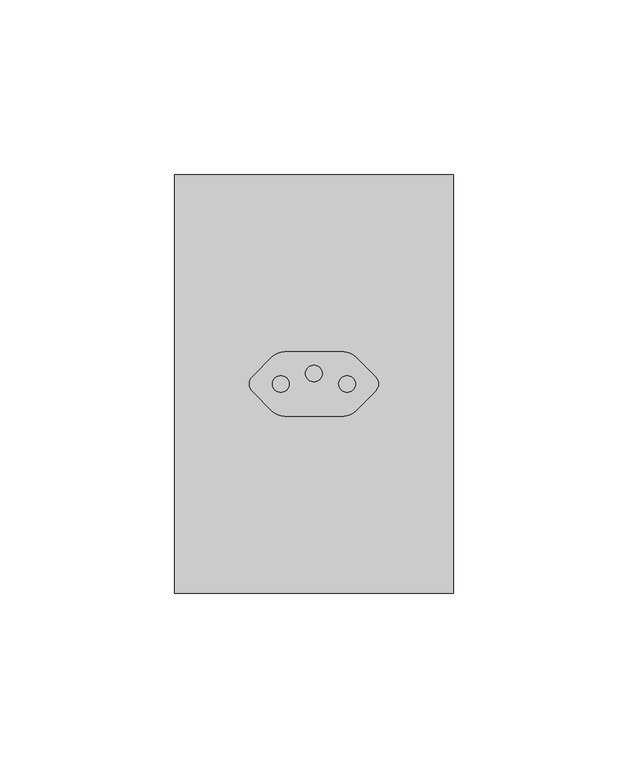
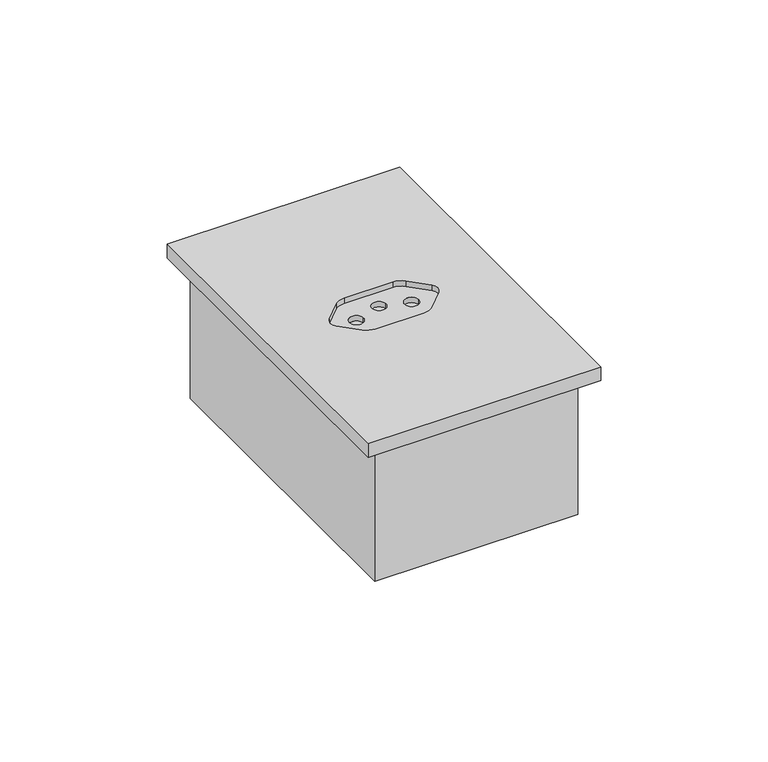
"""IFC4 building model written with IfcOpenShell, lengths in millimetres: proxy geometry, CAIXA VERTICE V7 : Tomada 20A 1s."""

from ifc_helpers import new_model, si_unit, frame, origin, place, context, project, spatial, polyline, circle_curve, faceted_brep, source, transform, mapped, element, save
from ifc_brep_helpers import plane_surface, revolved_surface, advanced_brep


def electrical_fixtures_88c6d9a2(model_context):
    return source(origin(), model_context, "Body", "SolidModel", [
        faceted_brep([(33.0, 247.0, -48.0), (33.0, 353.0, -48.0), (-33.0, 353.0, -48.0), (-33.0, 247.0, -48.0), (35.0, 355.0, -50.0), (35.0, 245.0, -50.0), (-35.0, 245.0, -50.0), (-35.0, 355.0, -50.0), (-35.0, 355.0, 0.0), (35.0, 355.0, 0.0), (-35.0, 245.0, 0.0), (35.0, 245.0, 0.0), (33.0, 353.0, 0.0), (33.0, 247.0, 0.0), (-33.0, 247.0, 0.0), (-33.0, 353.0, 0.0)], [[[0, 1, 2, 3]], [[4, 5, 6, 7]], [[4, 7, 8, 9]], [[8, 7, 6, 10]], [[10, 6, 5, 11]], [[11, 5, 4, 9]], [[9, 8, 10, 11], [12, 13, 14, 15]], [[13, 12, 1, 0]], [[14, 13, 0, 3]], [[15, 14, 3, 2]], [[12, 15, 2, 1]]]),
        advanced_brep(
        [(40.0, 360.0, 5.0), (-40.0, 360.0, 5.0), (-40.0, 240.0, 5.0), (40.0, 240.0, 5.0), (8.4215729, 290.75, 5.0), (-8.4215729, 290.75, 5.0), (-11.9571068, 292.2144661, 5.0), (-17.6213203, 297.8786797, 5.0), (-17.6213203, 302.1213203, 5.0), (-11.9571068, 307.7855339, 5.0), (-8.4215729, 309.25, 5.0), (8.4215729, 309.25, 5.0), (11.9571068, 307.7855339, 5.0), (17.6213203, 302.1213203, 5.0), (17.6213203, 297.8786797, 5.0), (11.9571068, 292.2144661, 5.0), (-40.0, 360.0, 0.0), (40.0, 360.0, 0.0), (40.0, 240.0, 0.0), (-40.0, 240.0, 0.0), (8.4215729, 290.75, 3.0), (11.9571068, 292.2144661, 3.0), (17.6213203, 297.8786797, 3.0), (17.6213203, 302.1213203, 3.0), (11.9571068, 307.7855339, 3.0), (8.4215729, 309.25, 3.0), (-8.4215729, 309.25, 3.0), (-11.9571068, 307.7855339, 3.0), (-17.6213203, 302.1213203, 3.0), (-17.6213203, 297.8786797, 3.0), (-11.9571068, 292.2144661, 3.0), (-8.4215729, 290.75, 3.0), (-7.1, 300.0, 3.0), (-11.9, 300.0, 3.0), (11.9, 300.0, 3.0), (7.1, 300.0, 3.0), (2.4, 303.0, 3.0), (-2.4, 303.0, 3.0), (-11.9, 300.0, 1.0), (-7.1, 300.0, 1.0), (7.1, 300.0, 1.0), (11.9, 300.0, 1.0), (-2.4, 303.0, 1.0), (2.4, 303.0, 1.0)],
        [
            (0, 1),
            (1, 2),
            (2, 3),
            (3, 0),
            (4, 5),
            (5, 6, circle_curve(frame((-8.4215729, 295.75, 5.0), z_axis=(0.0, 0.0, -1.0), x_axis=(-1.0, 0.0, 0.0)), 5.0)),
            (6, 7),
            (7, 8, circle_curve(frame((-15.5, 300.0, 5.0), z_axis=(0.0, 0.0, -1.0), x_axis=(-1.0, 0.0, 0.0)), 3.0)),
            (8, 9),
            (9, 10, circle_curve(frame((-8.4215729, 304.25, 5.0), z_axis=(0.0, 0.0, -1.0), x_axis=(-1.0, 0.0, 0.0)), 5.0)),
            (10, 11),
            (11, 12, circle_curve(frame((8.4215729, 304.25, 5.0), z_axis=(0.0, 0.0, -1.0), x_axis=(-1.0, 0.0, 0.0)), 5.0)),
            (12, 13),
            (13, 14, circle_curve(frame((15.5, 300.0, 5.0), z_axis=(0.0, 0.0, -1.0), x_axis=(-1.0, 0.0, 0.0)), 3.0)),
            (14, 15),
            (15, 4, circle_curve(frame((8.4215729, 295.75, 5.0), z_axis=(0.0, 0.0, -1.0), x_axis=(-1.0, 0.0, 0.0)), 5.0)),
            (16, 17),
            (17, 18),
            (18, 19),
            (19, 16),
            (0, 17),
            (16, 1),
            (19, 2),
            (18, 3),
            (20, 21, circle_curve(frame((8.4215729, 295.75, 3.0), z_axis=(0.0, 0.0, 1.0), x_axis=(-1.0, 0.0, 0.0)), 5.0)),
            (21, 22),
            (22, 23, circle_curve(frame((15.5, 300.0, 3.0), z_axis=(0.0, 0.0, 1.0), x_axis=(-1.0, 0.0, 0.0)), 3.0)),
            (23, 24),
            (24, 25, circle_curve(frame((8.4215729, 304.25, 3.0), z_axis=(0.0, 0.0, 1.0), x_axis=(-1.0, 0.0, 0.0)), 5.0)),
            (25, 26),
            (26, 27, circle_curve(frame((-8.4215729, 304.25, 3.0), z_axis=(0.0, 0.0, 1.0), x_axis=(-1.0, 0.0, 0.0)), 5.0)),
            (27, 28),
            (28, 29, circle_curve(frame((-15.5, 300.0, 3.0), z_axis=(0.0, 0.0, 1.0), x_axis=(-1.0, 0.0, 0.0)), 3.0)),
            (29, 30),
            (30, 31, circle_curve(frame((-8.4215729, 295.75, 3.0), z_axis=(0.0, 0.0, 1.0), x_axis=(-1.0, 0.0, 0.0)), 5.0)),
            (31, 20),
            (32, 33, circle_curve(frame((-9.5, 300.0, 3.0), z_axis=(0.0, 0.0, -1.0), x_axis=(1.0, 2.301812013077709e-12, 0.0)), 2.4)),
            (33, 32, circle_curve(frame((-9.5, 300.0, 3.0), z_axis=(0.0, 0.0, -1.0), x_axis=(1.0, 2.301812013077709e-12, 0.0)), 2.4)),
            (34, 35, circle_curve(frame((9.5, 300.0, 3.0), z_axis=(0.0, 0.0, -1.0), x_axis=(1.0, 2.301812013077709e-12, 0.0)), 2.4)),
            (35, 34, circle_curve(frame((9.5, 300.0, 3.0), z_axis=(0.0, 0.0, -1.0), x_axis=(1.0, 2.301812013077709e-12, 0.0)), 2.4)),
            (36, 37, circle_curve(frame((0.0, 303.0, 3.0), z_axis=(0.0, 0.0, -1.0), x_axis=(1.0, 2.301812013077709e-12, 0.0)), 2.4)),
            (37, 36, circle_curve(frame((0.0, 303.0, 3.0), z_axis=(0.0, 0.0, -1.0), x_axis=(1.0, 2.301812013077709e-12, 0.0)), 2.4)),
            (31, 5),
            (4, 20),
            (30, 6),
            (29, 7),
            (28, 8),
            (27, 9),
            (26, 10),
            (25, 11),
            (24, 12),
            (23, 13),
            (22, 14),
            (21, 15),
            (38, 39, circle_curve(frame((-9.5, 300.0, 1.0), z_axis=(0.0, 0.0, 1.0), x_axis=(1.0, 2.301812013077709e-12, 0.0)), 2.4)),
            (39, 38, circle_curve(frame((-9.5, 300.0, 1.0), z_axis=(0.0, 0.0, 1.0), x_axis=(1.0, 2.301812013077709e-12, 0.0)), 2.4)),
            (40, 41, circle_curve(frame((9.5, 300.0, 1.0), z_axis=(0.0, 0.0, 1.0), x_axis=(1.0, 2.301812013077709e-12, 0.0)), 2.4)),
            (41, 40, circle_curve(frame((9.5, 300.0, 1.0), z_axis=(0.0, 0.0, 1.0), x_axis=(1.0, 2.301812013077709e-12, 0.0)), 2.4)),
            (42, 43, circle_curve(frame((0.0, 303.0, 1.0), z_axis=(0.0, 0.0, 1.0), x_axis=(1.0, 2.301812013077709e-12, 0.0)), 2.4)),
            (43, 42, circle_curve(frame((0.0, 303.0, 1.0), z_axis=(0.0, 0.0, 1.0), x_axis=(1.0, 2.301812013077709e-12, 0.0)), 2.4)),
            (32, 39),
            (38, 33),
            (34, 41),
            (40, 35),
            (36, 43),
            (42, 37),
        ],
        [
            plane_surface(frame((-60.0, 360.0, 5.0), z_axis=(0.0, 0.0, 1.0), x_axis=(-1.0, 0.0, 0.0))),
            plane_surface(frame((-60.0, 360.0, 0.0), z_axis=(0.0, 0.0, -1.0), x_axis=(1.0, 0.0, 0.0))),
            plane_surface(frame((40.0, 360.0, 5.0), z_axis=(0.0, 1.0, 0.0), x_axis=(0.0, 0.0, -1.0))),
            plane_surface(frame((-40.0, 360.0, 5.0), z_axis=(-1.0, 0.0, 0.0), x_axis=(0.0, 0.0, -1.0))),
            plane_surface(frame((-40.0, 240.0, 5.0), z_axis=(0.0, -1.0, 0.0), x_axis=(0.0, 0.0, -1.0))),
            plane_surface(frame((40.0, 240.0, 5.0), z_axis=(1.0, 0.0, 0.0), x_axis=(0.0, 0.0, -1.0))),
            plane_surface(frame((3.4215729, 295.75, 3.0), z_axis=(0.0, 0.0, 1.0), x_axis=(0.0, 1.0, 0.0))),
            plane_surface(frame((-8.4215729, 290.75, 5.0), z_axis=(0.0, 1.0, 0.0), x_axis=(0.0, 0.0, -1.0))),
            revolved_surface(polyline([(-13.4215729, 295.75, 5.0), (-13.4215729, 295.75, 3.0)]), (-8.4215729, 295.75, 3.0), (0.0, 0.0, 1.0)),
            plane_surface(frame((-17.6213203, 297.8786797, 5.0), z_axis=(0.7071067811865045, 0.7071067811865905, 0.0), x_axis=(0.0, 0.0, -1.0))),
            revolved_surface(polyline([(-18.5, 300.0, 5.0), (-18.5, 300.0, 3.0)]), (-15.5, 300.0, 3.0), (0.0, 0.0, 1.0)),
            plane_surface(frame((-11.9571068, 307.7855339, 5.0), z_axis=(0.7071067811865515, -0.7071067811865437, 0.0), x_axis=(0.0, 0.0, -1.0))),
            revolved_surface(polyline([(-13.4215729, 304.25, 5.0), (-13.4215729, 304.25, 3.0)]), (-8.4215729, 304.25, 3.0), (0.0, 0.0, 1.0)),
            plane_surface(frame((8.4215729, 309.25, 5.0), z_axis=(0.0, -1.0, 0.0), x_axis=(0.0, 0.0, -1.0))),
            revolved_surface(polyline([(3.4215728999999993, 304.25, 5.0), (3.4215728999999993, 304.25, 3.0)]), (8.4215729, 304.25, 3.0), (0.0, 0.0, 1.0)),
            plane_surface(frame((17.6213203, 302.1213203, 5.0), z_axis=(-0.7071067811865307, -0.7071067811865643, 0.0), x_axis=(0.0, 0.0, -1.0))),
            revolved_surface(polyline([(12.5, 300.0, 5.0), (12.5, 300.0, 3.0)]), (15.5, 300.0, 3.0), (0.0, 0.0, 1.0)),
            plane_surface(frame((11.9571068, 292.2144661, 5.0), z_axis=(-0.7071067811865893, 0.7071067811865058, 0.0), x_axis=(0.0, 0.0, -1.0))),
            revolved_surface(polyline([(3.4215728999999993, 295.75, 5.0), (3.4215728999999993, 295.75, 3.0)]), (8.4215729, 295.75, 3.0), (0.0, 0.0, 1.0)),
            plane_surface(frame((-7.1, 300.0, 1.0), z_axis=(0.0, 0.0, 1.0), x_axis=(2.301812013077709e-12, -1.0, 0.0))),
            revolved_surface(polyline([(-7.1, 300.0000000000055, 3.0), (-7.1, 300.0000000000055, 1.0)]), (-9.5, 300.0, 1.0), (0.0, 0.0, 1.0)),
            revolved_surface(polyline([(11.9, 300.0000000000055, 3.0), (11.9, 300.0000000000055, 1.0)]), (9.5, 300.0, 5.0), (0.0, 0.0, 1.0)),
            revolved_surface(polyline([(2.4, 303.0000000000055, 3.0), (2.4, 303.0000000000055, 1.0)]), (0.0, 303.0, 5.0), (0.0, 0.0, 1.0)),
        ],
        [
            (0, [[1, 2, 3, 4], [5, 6, 7, 8, 9, 10, 11, 12, 13, 14, 15, 16]]),
            (1, [[17, 18, 19, 20]]),
            (2, [[-1, 21, -17, 22]]),
            (3, [[-2, -22, -20, 23]]),
            (4, [[-3, -23, -19, 24]]),
            (5, [[-4, -24, -18, -21]]),
            (6, [[25, 26, 27, 28, 29, 30, 31, 32, 33, 34, 35, 36], [37, 38], [39, 40], [41, 42]]),
            (7, [[-36, 43, -5, 44]]),
            (8, [[-35, 45, -6, -43]]),
            (9, [[-34, 46, -7, -45]]),
            (10, [[-33, 47, -8, -46]]),
            (11, [[-32, 48, -9, -47]]),
            (12, [[-31, 49, -10, -48]]),
            (13, [[-30, 50, -11, -49]]),
            (14, [[-29, 51, -12, -50]]),
            (15, [[-28, 52, -13, -51]]),
            (16, [[-27, 53, -14, -52]]),
            (17, [[-26, 54, -15, -53]]),
            (18, [[-25, -44, -16, -54]]),
            (19, [[55, 56]]),
            (19, [[57, 58]]),
            (19, [[59, 60]]),
            (20, [[-37, 61, -55, 62]]),
            (20, [[-38, -62, -56, -61]]),
            (21, [[-39, 63, -57, 64]]),
            (21, [[-40, -64, -58, -63]]),
            (22, [[-41, 65, -59, 66]]),
            (22, [[-42, -66, -60, -65]]),
        ],
    ),
    ])


if __name__ == "__main__":
    model = new_model("IFC4")
    model_context = context("Model", 3, world=origin())
    ifc_project = project(units=[si_unit("LENGTHUNIT", "METRE", prefix="MILLI")], contexts=[model_context])
    site = spatial("IfcSite", under=ifc_project)
    building = spatial("IfcBuilding", under=site)
    placement = place(None, origin())
    electrical_fixtures_shape = electrical_fixtures_88c6d9a2(model_context)
    element("IfcBuildingElementProxy", 1, Name="CAIXA VERTICE V7 : Tomada 20A 1s", ObjectType="CAIXA VERTICE V7 : Tomada 20A 1s", at=placement, inside=building, context=model_context, shape_type="MappedRepresentation", body=[
        mapped(electrical_fixtures_shape, transform((0.0, 0.0, 0.0), x_axis=(1.0, 0.0, 0.0), y_axis=(0.0, 1.0, 0.0), z_axis=(0.0, 0.0, 1.0))),
    ])
    save(model, "model.ifc")

# Revit data of these elements
# Type "CAIXA VERTICE V7 : Tomada 20A 1s"
#   URL = "www.facebook.com/verticetreinamentos"
#   SEÇÃO [instance default] = ""
#   Rotação [instance default] = 0.00°
#   LARGURA DA TAMPA = 0.08 m
#   BORDA = 0.01 m
#   ALTURA DE INSTALAÇÃO [instance default] = 1.10 m
#   Distância Anotação [instance default] = 0.0015 m
#   ALTURA DA TAMPA = 0.12 m
#   Vertical [instance default] = yes
#   VER SEÇÃO [instance default] = no
#   SHADE ESQ [instance default] = no
#   SHADE DIR [instance default] = yes
#   HORIZONTAL [instance default] = no
#   ANDAR COM A LEGENDA [instance default] = 0
#   Material Tampa [instance default] = Plástico, branco opaco
#   Caixa = element 1798517
#   Anotação = element 1798531
#   Default Elevation = 0
# Element 1 (IfcBuildingElementProxy, "CAIXA VERTICE V7 : Tomada 20A 1s")
#   ALTURA DE INSTALAÇÃO = 0.30 m
#   SHADE DIR = no
#   Materials on its faces: "Plástico, branco opaco"
# Materials
#   "Plástico, branco opaco": class "Plástico", colour RGB 120 120 120, transparency 0, Description = "Plastic, generic, opaque white", Cost = 0
